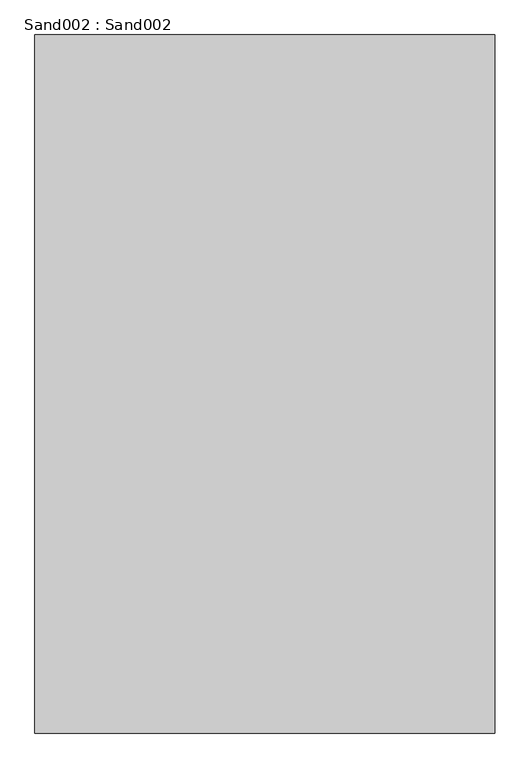
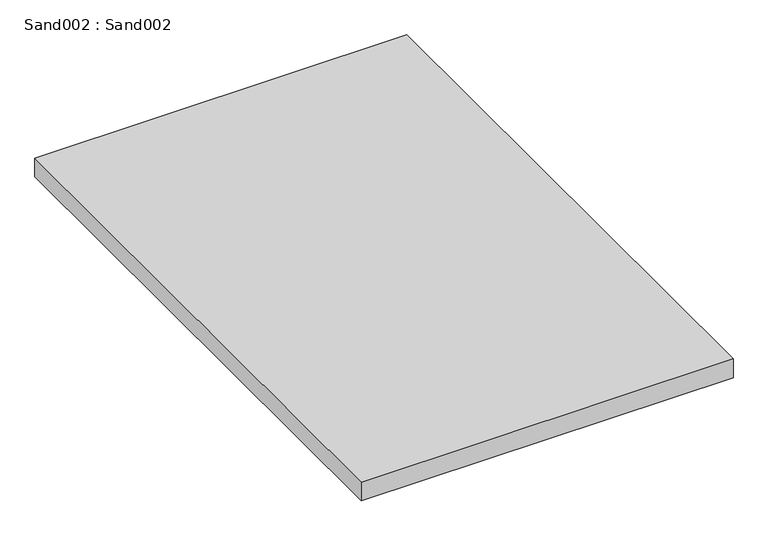
"""IFC4 building model written with IfcOpenShell, lengths in millimetres: proxy geometry, Sand002 : Sand002."""

from ifc_helpers import new_model, si_unit, frame, origin, place, context, project, spatial, polyline, outline, extrude, source, transform, mapped, element, save


def sand002_sand002_d9a6552e(model_context):
    return source(origin(), model_context, "Body", "SweptSolid", [
        extrude(outline(polyline([(-10250.8737014, 7982.1529359), (-11568.4300809, 7982.1529359), (-11568.4300809, 9982.1529359), (-10250.8737014, 9982.1529359), (-10250.8737014, 7982.1529359)])), frame((0.0, 0.0, 32397.0602473), z_axis=(0.0, 0.0, 1.0), x_axis=(1.0, 0.0, 0.0)), (0.0, 0.0, 1.0), 70.2358801),
    ])


if __name__ == "__main__":
    model = new_model("IFC4")
    model_context = context("Model", 3, world=origin())
    ifc_project = project(units=[si_unit("LENGTHUNIT", "METRE", prefix="MILLI")], contexts=[model_context])
    site = spatial("IfcSite", under=ifc_project)
    building = spatial("IfcBuilding", under=site)
    placement = place(None, origin())
    sand002_sand002_shape = sand002_sand002_d9a6552e(model_context)
    element("IfcBuildingElementProxy", 1, Name="Sand002 : Sand002", ObjectType="Sand002 : Sand002", at=placement, inside=building, context=model_context, shape_type="MappedRepresentation", body=[
        mapped(sand002_sand002_shape, transform((0.0, 0.0, 0.0), x_axis=(1.0, 0.0, 0.0), y_axis=(0.0, 1.0, 0.0), z_axis=(0.0, 0.0, 1.0))),
    ])
    save(model, "model.ifc")

# Revit data of these elements
# Type "Sand002 : Sand002"
#   NameOverride = "Sand002"
# Element 1 (IfcBuildingElementProxy, "Sand002 : Sand002")
#   Materials on its faces: "2\" SAND LAYER"
# Materials
#   "2\" SAND LAYER": class "Unassigned", colour RGB 239 206 153, transparency 0, Cost = 0
